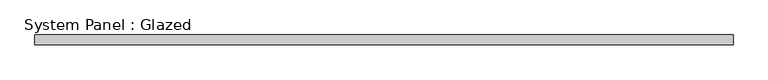
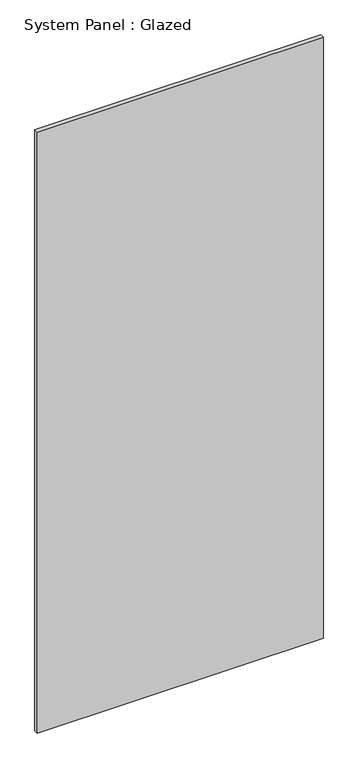
"""IFC4 building model written with IfcOpenShell, lengths in millimetres: plate geometry, System Panel : Glazed."""

import ifcopenshell
import ifcopenshell.guid

model = None  # the IFC model being written
_history = None  # IfcOwnerHistory: only IFC2X3 demands one
_inside = {}  # id of a spatial element -> (the spatial element, [elements in it])
_under = {}  # id of a project, library or spatial element -> (it, [spatial elements below it])
_declared = {}  # id of a project -> (the project, [libraries it declares])
_typed = {}  # id of a type object -> (the type object, [elements of that type])
_made_of = {}  # id of a material, layer set ... -> (it, [elements and type objects made of it])


def new_model(schema):
    """Start an empty IFC model of exactly this schema.

    Asked for "IFC4X3", IfcOpenShell would pick the latest addendum, in which some entities
    have other attributes; the version numbers below select the first issue.
    IFC2X3 requires an IfcOwnerHistory on every rooted entity: one is made here for all.
    """
    global model, _history
    if schema == "IFC4X3":
        model = ifcopenshell.file(schema_version=(4, 3, 0, 0))
    else:
        model = ifcopenshell.file(schema=schema)
    _inside.clear()
    _under.clear()
    _declared.clear()
    _typed.clear()
    _made_of.clear()
    _history = None
    if model.schema == "IFC2X3":
        org = make("IfcOrganization", Name="unknown")
        user = make(
            "IfcPersonAndOrganization",
            ThePerson=make("IfcPerson", FamilyName="unknown"),
            TheOrganization=org,
        )
        app = make(
            "IfcApplication",
            ApplicationDeveloper=org,
            Version="unknown",
            ApplicationFullName="unknown",
            ApplicationIdentifier="unknown",
        )
        _history = make(
            "IfcOwnerHistory",
            OwningUser=user,
            OwningApplication=app,
            ChangeAction="ADDED",
            CreationDate=0,
        )
    return model


def make(cls, **values):
    """One entity of the class cls with the attributes given. An attribute that is None is left unset."""
    return model.create_entity(
        cls, **{name: value for name, value in values.items() if value is not None}
    )


def rooted(cls, **values):
    """An entity with a GlobalId (a new one), such as an element, a storey or a relation."""
    return make(cls, GlobalId=ifcopenshell.guid.new(), OwnerHistory=_history, **values)


def si_unit(unit_type, name, prefix=None):
    """IfcSIUnit, for example si_unit("LENGTHUNIT", "METRE", prefix="MILLI")."""
    return make("IfcSIUnit", UnitType=unit_type, Prefix=prefix, Name=name)


def assignment(units):
    """IfcUnitAssignment: the units of a project."""
    return None if units is None else make("IfcUnitAssignment", Units=units)


def point(xyz):
    """IfcCartesianPoint."""
    return None if xyz is None else make("IfcCartesianPoint", Coordinates=xyz)


def direction(xyz):
    """IfcDirection."""
    return None if xyz is None else make("IfcDirection", DirectionRatios=xyz)


def frame(location, z_axis=None, x_axis=None):
    """IfcAxis2Placement3D, a coordinate frame: its origin and axes. An axis left out is left unset."""
    return make(
        "IfcAxis2Placement3D",
        Location=point(location),
        Axis=direction(z_axis),
        RefDirection=direction(x_axis),
    )


def origin():
    """The frame at (0, 0, 0) with its axes left unset."""
    return frame((0.0, 0.0, 0.0))


def origin_with_axes():
    """The frame at (0, 0, 0) with the z axis (0, 0, 1) and the x axis (1, 0, 0) written out."""
    return frame((0.0, 0.0, 0.0), z_axis=(0.0, 0.0, 1.0), x_axis=(1.0, 0.0, 0.0))


def place(relative_to, where):
    """IfcLocalPlacement: puts the frame where relative to a parent placement (None: the world)."""
    return make(
        "IfcLocalPlacement", PlacementRelTo=relative_to, RelativePlacement=where
    )


def context(
    kind, dimensions, precision=None, world=None, true_north=None, identifier=None
):
    """IfcGeometricRepresentationContext, for example the 3D "Model" context."""
    return make(
        "IfcGeometricRepresentationContext",
        ContextIdentifier=identifier,
        ContextType=kind,
        CoordinateSpaceDimension=dimensions,
        Precision=precision,
        WorldCoordinateSystem=world,
        TrueNorth=true_north,
    )


def project(units=None, contexts=None):
    """IfcProject with its units and contexts."""
    return rooted(
        "IfcProject",
        Name="project",
        RepresentationContexts=contexts,
        UnitsInContext=assignment(units),
    )


def spatial(cls, under=None, at=None, **own):
    """A site, building, storey or space (cls), placed at a placement, below another one or the project."""
    s = rooted(cls, ObjectPlacement=at, **own)
    if under is not None:
        _under.setdefault(under.id(), (under, []))[1].append(s)
    return s


def polyline(points):
    """IfcPolyline through the points."""
    return make("IfcPolyline", Points=[point(p) for p in points])


def outline(outer, holes=None, kind="AREA"):
    """IfcArbitraryClosedProfileDef: a profile drawn as a closed curve; with holes, ...WithVoids."""
    if holes is None:
        return make("IfcArbitraryClosedProfileDef", ProfileType=kind, OuterCurve=outer)
    return make(
        "IfcArbitraryProfileDefWithVoids",
        ProfileType=kind,
        OuterCurve=outer,
        InnerCurves=holes,
    )


def extrude(swept, where, along, depth):
    """IfcExtrudedAreaSolid: the profile swept, set in the frame where, extruded along a direction by depth."""
    return make(
        "IfcExtrudedAreaSolid",
        SweptArea=swept,
        Position=where,
        ExtrudedDirection=direction(along),
        Depth=depth,
    )


def shape(context_of_items, identifier, shape_type, items):
    """IfcShapeRepresentation: the items that make up one representation, for example the "Body"."""
    return make(
        "IfcShapeRepresentation",
        ContextOfItems=context_of_items,
        RepresentationIdentifier=identifier,
        RepresentationType=shape_type,
        Items=items,
    )


def source(mapping_origin, context_of_items, identifier, shape_type, items):
    """IfcRepresentationMap: a shape defined once, which mapped items show again and again."""
    return make(
        "IfcRepresentationMap",
        MappingOrigin=mapping_origin,
        MappedRepresentation=shape(context_of_items, identifier, shape_type, items),
    )


def transform(
    local_origin,
    x_axis=None,
    y_axis=None,
    z_axis=None,
    scale=None,
    scale2=None,
    scale3=None,
    uniform=True,
):
    """IfcCartesianTransformationOperator3D, or its non-uniform kind. x_axis, y_axis, z_axis: its Axis1, 2, 3."""
    if uniform:
        return make(
            "IfcCartesianTransformationOperator3D",
            Axis1=direction(x_axis),
            Axis2=direction(y_axis),
            LocalOrigin=point(local_origin),
            Scale=scale,
            Axis3=direction(z_axis),
        )
    return make(
        "IfcCartesianTransformationOperator3DnonUniform",
        Axis1=direction(x_axis),
        Axis2=direction(y_axis),
        LocalOrigin=point(local_origin),
        Scale=scale,
        Axis3=direction(z_axis),
        Scale2=scale2,
        Scale3=scale3,
    )


def mapped(mapping_source, mapping_target):
    """IfcMappedItem: shows the shape of a source again, moved by a transform."""
    return make(
        "IfcMappedItem", MappingSource=mapping_source, MappingTarget=mapping_target
    )


def made_of(thing, what):
    """Note that an element or type object is made of a material, layer set ...; save() writes the relation."""
    if what is not None:
        _made_of.setdefault(what.id(), (what, []))[1].append(thing)
    return thing


def element(
    cls,
    number,
    at=None,
    inside=None,
    cuts=None,
    type_object=None,
    material=None,
    context=None,
    identifier="Body",
    shape_type=None,
    held_by="IfcProductDefinitionShape",
    body=None,
    shapes=None,
    **own,
):
    """One element of the class cls, such as IfcWall. Its Tag is "e" and its number.

    at: its placement. inside: the storey or other place that contains it. cuts: it is an
    opening in that element (IfcRelVoidsElement). A single representation is given by context,
    identifier, shape_type and body (its items); several are given by shapes. held_by: the class
    of the entity that holds the representations. save() writes the other relations.
    """
    e = rooted(cls, Tag="e%d" % number, ObjectPlacement=at, **own)
    if body is not None:
        shapes = [shape(context, identifier, shape_type, body)]
    if shapes is not None:
        e.Representation = make(held_by, Representations=shapes)
    if inside is not None:
        _inside.setdefault(inside.id(), (inside, []))[1].append(e)
    if cuts is not None:
        rooted(
            "IfcRelVoidsElement", RelatingBuildingElement=cuts, RelatedOpeningElement=e
        )
    if type_object is not None:
        _typed.setdefault(type_object.id(), (type_object, []))[1].append(e)
    return made_of(e, material)


def aggregate(whole, parts):
    """IfcRelAggregates: a whole, such as a stair, and the parts it consists of."""
    return rooted("IfcRelAggregates", RelatingObject=whole, RelatedObjects=parts)


def save(model, path):
    """Write the relations noted so far, then the file.

    IfcRelAggregates (storeys below a building ...), IfcRelContainedInSpatialStructure (elements
    in a storey), IfcRelDefinesByType, IfcRelAssociatesMaterial and IfcRelDeclares: one each for
    every whole, place, type object, material and project.
    """
    for whole, parts in _under.values():
        aggregate(whole, parts)
    for where, things in _inside.values():
        rooted(
            "IfcRelContainedInSpatialStructure",
            RelatedElements=things,
            RelatingStructure=where,
        )
    for kind, things in _typed.values():
        rooted("IfcRelDefinesByType", RelatedObjects=things, RelatingType=kind)
    for what, things in _made_of.values():
        rooted("IfcRelAssociatesMaterial", RelatedObjects=things, RelatingMaterial=what)
    for by, libraries in _declared.values():
        rooted("IfcRelDeclares", RelatingContext=by, RelatedDefinitions=libraries)
    model.write(path)


def system_panel_glazed_e467a615(model_context):
    return source(origin(), model_context, "Body", "SweptSolid", [
        extrude(outline(polyline([(890.0, 24.5), (-890.0, 24.5), (-890.0, 49.5), (890.0, 49.5), (890.0, 24.5)])), origin_with_axes(), (0.0, 0.0, 1.0), 3950.0),
    ])


if __name__ == "__main__":
    model = new_model("IFC4")
    model_context = context("Model", 3, world=origin())
    ifc_project = project(units=[si_unit("LENGTHUNIT", "METRE", prefix="MILLI")], contexts=[model_context])
    site = spatial("IfcSite", under=ifc_project)
    building = spatial("IfcBuilding", under=site)
    placement = place(None, origin())
    system_panel_glazed_shape = system_panel_glazed_e467a615(model_context)
    element("IfcPlate", 1, ObjectType="System Panel : Glazed", at=placement, inside=building, context=model_context, shape_type="MappedRepresentation", body=[
        mapped(system_panel_glazed_shape, transform((0.0, 0.0, 0.0), x_axis=(1.0, 0.0, 0.0), y_axis=(0.0, 1.0, 0.0), z_axis=(0.0, 0.0, 1.0))),
    ])
    save(model, "model.ifc")

# Revit data of these elements
# Type "System Panel : Glazed"
#   Keynote = "H11"
#   Construction Type Id = "GSP4R"
#   Analytic Construction = "1/8 in Pilkington single glazing"
#   Visual Light Transmittance = 0.9
#   Solar Heat Gain Coefficient = 0.86
#   Heat Transfer Coefficient (U) = 6.7069 W/(m²·K)
#   Define Thermal Properties by = 1
# Element 1 (IfcPlate, "System Panel : Glazed")
#   Materials on its faces: "Glass"
# Materials
#   "Glass": class "Glass", colour RGB 0 128 192, transparency 0.9, Description = "Soda Lime Glass", Cost = 0
